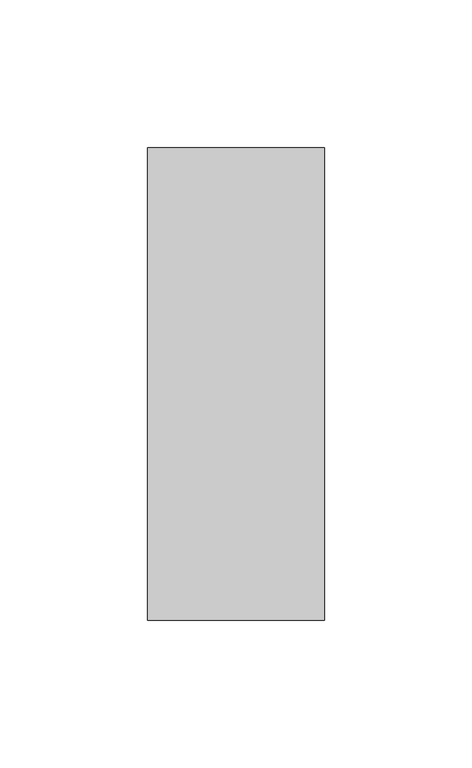
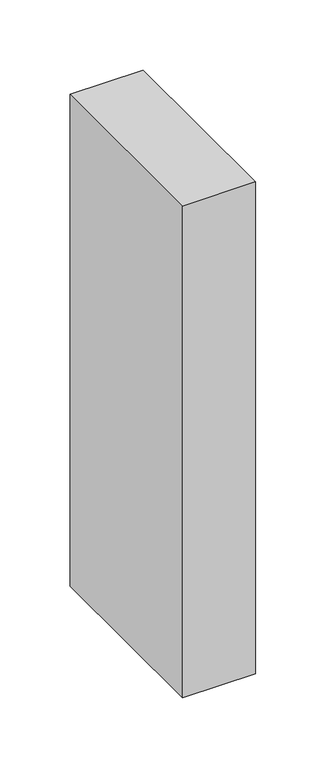
"""IFC4 building model written with IfcOpenShell, lengths in millimetres: column geometry, Madeira de lei-Coluna : Pontalete 6X16cm."""

from ifc_helpers import new_model, si_unit, frame, origin, place, context, project, spatial, polyline, outline, extrude, source, transform, mapped, element, save


def column_4d3918cc(model_context):
    return source(origin(), model_context, "Body", "SweptSolid", [
        extrude(outline(polyline([(30.0, 80.0), (30.0, -80.0), (-30.0, -80.0), (-30.0, 80.0), (30.0, 80.0)])), frame((0.0, 0.0, 4460.0), z_axis=(0.0, 0.0, 1.0), x_axis=(1.0, 0.0, 0.0)), (0.0, 0.0, 1.0), 426.9),
    ])


if __name__ == "__main__":
    model = new_model("IFC4")
    model_context = context("Model", 3, world=origin())
    ifc_project = project(units=[si_unit("LENGTHUNIT", "METRE", prefix="MILLI")], contexts=[model_context])
    site = spatial("IfcSite", under=ifc_project)
    building = spatial("IfcBuilding", under=site)
    placement = place(None, origin())
    column_shape = column_4d3918cc(model_context)
    element("IfcColumn", 1, ObjectType="Madeira de lei-Coluna : Pontalete 6X16cm", at=placement, inside=building, context=model_context, shape_type="MappedRepresentation", body=[
        mapped(column_shape, transform((0.0, 0.0, 0.0), x_axis=(1.0, 0.0, 0.0), y_axis=(0.0, 1.0, 0.0), z_axis=(0.0, 0.0, 1.0))),
    ])
    save(model, "model.ifc")

# Revit data of these elements
# Type "Madeira de lei-Coluna : Pontalete 6X16cm"
#   A = 0.01952 m²
#   b = 0.06 m
#   d = 0.16 m
#   Structural Material [instance default] = none
#   Assembly Code = ""
# Element 1 (IfcColumn, "Madeira de lei-Coluna : Pontalete 6X16cm")
#   Structural Material = .MADEIRAMENTO
#   Materials on its faces: ".MADEIRAMENTO"
# Materials
#   ".MADEIRAMENTO": class ".CC_MADEIRAS", colour RGB 212 179 113, transparency 0, Cost = 0
